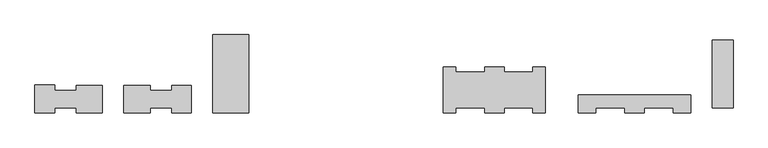
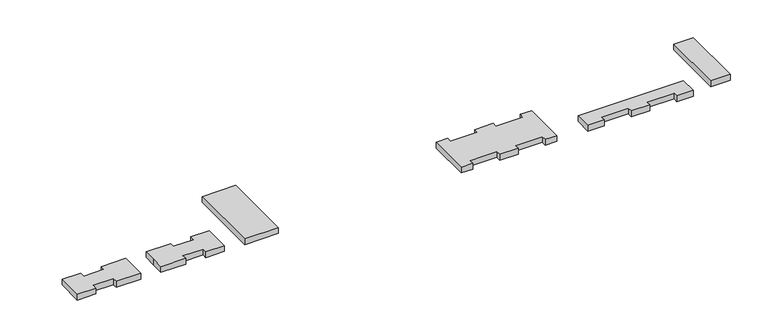
"""IFC4 building model written with IfcOpenShell, lengths in millimetres: geographic element geometry, 6th sty Planting : 6th sty Planting."""

from ifc_helpers import new_model, si_unit, frame, origin, place, context, project, spatial, polyline, outline, extrude, source, transform, mapped, element, save


def geographic_element_353681dd(model_context):
    return source(origin(), model_context, "Body", "SweptSolid", [
        extrude(outline(polyline([(6642.7196734, 3650.1819645), (6642.7196734, 3280.1819645), (8142.7196734, 3280.1819645), (8142.7196734, 3630.1819645), (9962.7196734, 3630.1819645), (9962.7196734, 2655.2285337), (9962.7196734, 1710.0), (8142.7196734, 1710.0), (8142.7196734, 2060.0), (6642.7196734, 2060.0), (6642.7196734, 1710.0), (5279.4029609, 1710.0), (5279.4029609, 3650.1819645), (6642.7196734, 3650.1819645)])), frame((0.0, 0.0, 143070.0), z_axis=(0.0, 0.0, 1.0), x_axis=(1.0, 0.0, 0.0)), (0.0, 0.0, 1.0), 450.0),
        extrude(outline(polyline([(11462.7196734, 2643.2526171), (11462.7196734, 3630.1819645), (13282.7833134, 3630.1819645), (13282.7833134, 3280.1819645), (14782.7833134, 3280.1819645), (14782.7833134, 3630.1819645), (16145.4393469, 3630.1819645), (16145.4393469, 1710.0), (14782.7833134, 1710.0), (14782.7833134, 2060.0), (13282.7833134, 2060.0), (13282.7833134, 1710.0), (11462.7196734, 1710.0), (11462.7196734, 2643.2526171)])), frame((0.0, 0.0, 143070.0), z_axis=(0.0, 0.0, 1.0), x_axis=(1.0, 0.0, 0.0)), (0.0, 0.0, 1.0), 450.0),
        extrude(outline(polyline([(20149.8343294, 7159.9624711), (20149.8343294, 1710.0), (17645.4393469, 1710.0), (17645.4393469, 7159.9624711), (20149.8343294, 7159.9624711)])), frame((0.0, 0.0, 143070.0), z_axis=(0.0, 0.0, 1.0), x_axis=(1.0, 0.0, 0.0)), (0.0, 0.0, 1.0), 450.0),
        extrude(outline(polyline([(33675.2145751, 4925.0), (34525.2145751, 4925.0), (34525.2145751, 4575.0), (36525.2145751, 4575.0), (36525.2145751, 4925.0), (37895.2145752, 4925.0), (37895.2145752, 4575.0), (39895.2145752, 4575.0), (39895.2145752, 4925.0), (40745.0744751, 4925.0), (40745.0744751, 1710.0), (39895.2145752, 1710.0), (39895.2145752, 2060.0), (37895.2145752, 2060.0), (37895.2145752, 1710.0), (36525.2145751, 1710.0), (36525.2145751, 2060.0), (34525.2145751, 2060.0), (34525.2145751, 1710.0), (33675.2145751, 1710.0), (33675.2145751, 4925.0)])), frame((0.0, 0.0, 143070.0), z_axis=(0.0, 0.0, 1.0), x_axis=(1.0, 0.0, 0.0)), (0.0, 0.0, 1.0), 450.0),
        extrude(outline(polyline([(43045.0744751, 2950.0), (50845.4009563, 2950.0), (50845.4009563, 1710.0), (49630.2377158, 1710.0), (49630.2377158, 2060.0), (47630.2377158, 2060.0), (47630.2377158, 1710.0), (46260.2377157, 1710.0), (46260.2377157, 2060.0), (44260.2377157, 2060.0), (44260.2377157, 1710.0), (43045.0744751, 1710.0), (43045.0744751, 2950.0)])), frame((0.0, 0.0, 143070.0), z_axis=(0.0, 0.0, 1.0), x_axis=(1.0, 0.0, 0.0)), (0.0, 0.0, 1.0), 450.0),
        extrude(outline(polyline([(53800.9876732, 6800.0), (53800.9876732, 2060.0), (52345.4009563, 2060.0), (52345.4009563, 6800.0), (53800.9876732, 6800.0)])), frame((0.0, 0.0, 143070.0), z_axis=(0.0, 0.0, 1.0), x_axis=(1.0, 0.0, 0.0)), (0.0, 0.0, 1.0), 450.0),
    ])


if __name__ == "__main__":
    model = new_model("IFC4")
    model_context = context("Model", 3, world=origin())
    ifc_project = project(units=[si_unit("LENGTHUNIT", "METRE", prefix="MILLI")], contexts=[model_context])
    site = spatial("IfcSite", under=ifc_project)
    building = spatial("IfcBuilding", under=site)
    placement = place(None, origin())
    geographic_element_shape = geographic_element_353681dd(model_context)
    element("IfcGeographicElement", 1, ObjectType="6th sty Planting : 6th sty Planting", at=placement, inside=building, context=model_context, shape_type="MappedRepresentation", body=[
        mapped(geographic_element_shape, transform((0.0, 0.0, 0.0), x_axis=(1.0, 0.0, 0.0), y_axis=(0.0, 1.0, 0.0), z_axis=(0.0, 0.0, 1.0))),
    ])
    save(model, "model.ifc")

# Revit data of these elements
# Type "6th sty Planting : 6th sty Planting"
#   Height = 0
# Element 1 (IfcGeographicElement, "6th sty Planting : 6th sty Planting")
#   Materials on its faces: "Planting"
# Materials
#   "Planting": class "Unassigned", colour RGB 128 255 0, transparency 0.52, Cost = 0
